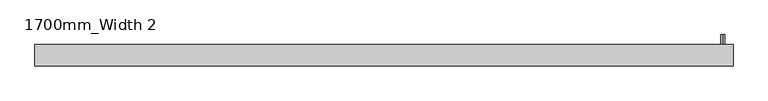
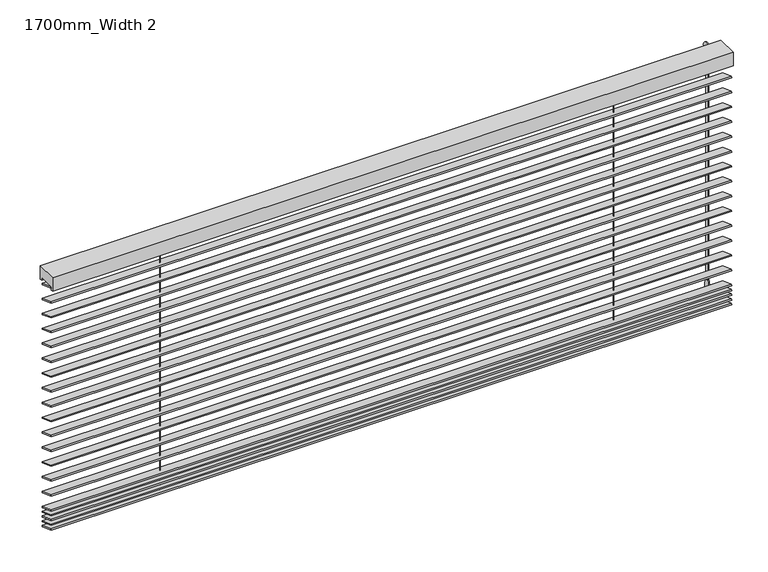
"""IFC4 building model written with IfcOpenShell, lengths in millimetres: proxy geometry, Specialty_Equipment_Venetian_Blind_Half_Down : 1700mm_Width 2."""

from ifc_helpers import new_model, si_unit, point, frame, frame_2d, origin, place, context, project, spatial, polyline, circle_curve, ellipse_curve, trimmed, segment, composite_curve, outline, extrude, source, transform, mapped, element, save
from ifc_brep_helpers import plane_surface, cylinder_surface, revolved_surface, advanced_brep


def proxy_1700mm_width_2_f283f02f(model_context):
    return source(origin(), model_context, "Body", "SolidModel", [
        extrude(outline(polyline([(0.0, 40.0), (1680.0, 40.0), (1680.0, 0.0), (0.0, 0.0), (0.0, 40.0)])), frame((-689.5079376, -65.0532351, 1447.7279746), z_axis=(0.0, 0.3420201433256684, 0.9396926207859085), x_axis=(1.0, 0.0, 0.0)), (0.0, 0.0, 1.0), 3.0625345),
        extrude(outline(polyline([(0.0, 40.0), (1680.0, 40.0), (1680.0, 0.0), (0.0, 0.0), (0.0, 40.0)])), frame((-689.5079376, -65.0532351, 1459.9116214), z_axis=(0.0, 0.3420201433256684, 0.9396926207859085), x_axis=(1.0, 0.0, 0.0)), (0.0, 0.0, 1.0), 3.0625345),
        extrude(outline(polyline([(0.0, 40.0), (1680.0, 40.0), (1680.0, 0.0), (0.0, 0.0), (0.0, 40.0)])), frame((-689.5079376, -65.0532351, 1472.7202682), z_axis=(0.0, 0.3420201433256684, 0.9396926207859085), x_axis=(1.0, 0.0, 0.0)), (0.0, 0.0, 1.0), 3.0625345),
        extrude(outline(polyline([(0.0, 40.0), (1680.0, 40.0), (1680.0, 0.0), (0.0, 0.0), (0.0, 40.0)])), frame((-689.5079376, -65.0532351, 1484.903915), z_axis=(0.0, 0.3420201433256684, 0.9396926207859085), x_axis=(1.0, 0.0, 0.0)), (0.0, 0.0, 1.0), 3.0625345),
        extrude(outline(polyline([(0.0, 40.0), (1680.0, 40.0), (1680.0, 0.0), (0.0, 0.0), (0.0, 40.0)])), frame((-689.5079376, -65.0532351, 2040.2125618), z_axis=(0.0, 0.3420201433256684, 0.9396926207859085), x_axis=(1.0, 0.0, 0.0)), (0.0, 0.0, 1.0), 3.0625345),
        extrude(outline(polyline([(0.0, 40.0), (1680.0, 40.0), (1680.0, 0.0), (0.0, 0.0), (0.0, 40.0)])), frame((-689.5079376, -65.0532351, 2001.4625618), z_axis=(0.0, 0.3420201433256684, 0.9396926207859085), x_axis=(1.0, 0.0, 0.0)), (0.0, 0.0, 1.0), 3.0625345),
        extrude(outline(polyline([(0.0, 40.0), (1680.0, 40.0), (1680.0, 0.0), (0.0, 0.0), (0.0, 40.0)])), frame((-689.5079376, -65.0532351, 1962.7125618), z_axis=(0.0, 0.3420201433256684, 0.9396926207859085), x_axis=(1.0, 0.0, 0.0)), (0.0, 0.0, 1.0), 3.0625345),
        extrude(outline(polyline([(0.0, 40.0), (1680.0, 40.0), (1680.0, 0.0), (0.0, 0.0), (0.0, 40.0)])), frame((-689.5079376, -65.0532351, 1923.9625618), z_axis=(0.0, 0.3420201433256684, 0.9396926207859085), x_axis=(1.0, 0.0, 0.0)), (0.0, 0.0, 1.0), 3.0625345),
        extrude(outline(polyline([(0.0, 40.0), (1680.0, 40.0), (1680.0, 0.0), (0.0, 0.0), (0.0, 40.0)])), frame((-689.5079376, -65.0532351, 1885.2125618), z_axis=(0.0, 0.3420201433256684, 0.9396926207859085), x_axis=(1.0, 0.0, 0.0)), (0.0, 0.0, 1.0), 3.0625345),
        extrude(outline(polyline([(0.0, 40.0), (1680.0, 40.0), (1680.0, 0.0), (0.0, 0.0), (0.0, 40.0)])), frame((-689.5079376, -65.0532351, 1846.4625618), z_axis=(0.0, 0.3420201433256684, 0.9396926207859085), x_axis=(1.0, 0.0, 0.0)), (0.0, 0.0, 1.0), 3.0625345),
        extrude(outline(polyline([(0.0, 40.0), (1680.0, 40.0), (1680.0, 0.0), (0.0, 0.0), (0.0, 40.0)])), frame((-689.5079376, -65.0532351, 1807.7125618), z_axis=(0.0, 0.3420201433256684, 0.9396926207859085), x_axis=(1.0, 0.0, 0.0)), (0.0, 0.0, 1.0), 3.0625345),
        extrude(outline(polyline([(0.0, 40.0), (1680.0, 40.0), (1680.0, 0.0), (0.0, 0.0), (0.0, 40.0)])), frame((-689.5079376, -65.0532351, 1768.9625618), z_axis=(0.0, 0.3420201433256684, 0.9396926207859085), x_axis=(1.0, 0.0, 0.0)), (0.0, 0.0, 1.0), 3.0625345),
        extrude(outline(polyline([(0.0, 40.0), (1680.0, 40.0), (1680.0, 0.0), (0.0, 0.0), (0.0, 40.0)])), frame((-689.5079376, -65.0532351, 1730.2125618), z_axis=(0.0, 0.3420201433256684, 0.9396926207859085), x_axis=(1.0, 0.0, 0.0)), (0.0, 0.0, 1.0), 3.0625345),
        extrude(outline(polyline([(0.0, 40.0), (1680.0, 40.0), (1680.0, 0.0), (0.0, 0.0), (0.0, 40.0)])), frame((-689.5079376, -65.0532351, 1691.4625618), z_axis=(0.0, 0.3420201433256684, 0.9396926207859085), x_axis=(1.0, 0.0, 0.0)), (0.0, 0.0, 1.0), 3.0625345),
        extrude(outline(polyline([(0.0, 40.0), (1680.0, 40.0), (1680.0, 0.0), (0.0, 0.0), (0.0, 40.0)])), frame((-689.5079376, -65.0532351, 1652.7125618), z_axis=(0.0, 0.3420201433256684, 0.9396926207859085), x_axis=(1.0, 0.0, 0.0)), (0.0, 0.0, 1.0), 3.0625345),
        extrude(outline(polyline([(0.0, 40.0), (1680.0, 40.0), (1680.0, 0.0), (0.0, 0.0), (0.0, 40.0)])), frame((-689.5079376, -65.0532351, 1613.9625618), z_axis=(0.0, 0.3420201433256684, 0.9396926207859085), x_axis=(1.0, 0.0, 0.0)), (0.0, 0.0, 1.0), 3.0625345),
        extrude(outline(polyline([(0.0, 40.0), (1680.0, 40.0), (1680.0, 0.0), (0.0, 0.0), (0.0, 40.0)])), frame((-689.5079376, -65.0532351, 1575.2125618), z_axis=(0.0, 0.3420201433256684, 0.9396926207859085), x_axis=(1.0, 0.0, 0.0)), (0.0, 0.0, 1.0), 3.0625345),
        extrude(outline(polyline([(0.0, 40.0), (1680.0, 40.0), (1680.0, 0.0), (0.0, 0.0), (0.0, 40.0)])), frame((-689.5079376, -65.0532351, 1536.4625618), z_axis=(0.0, 0.3420201433256684, 0.9396926207859085), x_axis=(1.0, 0.0, 0.0)), (0.0, 0.0, 1.0), 3.0625345),
        extrude(outline(polyline([(0.0, 40.0), (1680.0, 40.0), (1680.0, 0.0), (0.0, 0.0), (0.0, 40.0)])), frame((-689.5079376, -65.0532351, 1497.7125618), z_axis=(0.0, 0.3420201433256684, 0.9396926207859085), x_axis=(1.0, 0.0, 0.0)), (0.0, 0.0, 1.0), 3.0625345),
        extrude(outline(polyline([(0.0, 40.0), (1680.0, 40.0), (1680.0, 0.0), (0.0, 0.0), (0.0, 40.0)])), frame((-689.5079376, -65.0532351, 2078.9625618), z_axis=(0.0, 0.3420201433256684, 0.9396926207859085), x_axis=(1.0, 0.0, 0.0)), (0.0, 0.0, 1.0), 3.0625345),
        extrude(outline(composite_curve([segment(trimmed(circle_curve(frame_2d((-409.5079376, -45.2119342)), 0.5), [point((-410.0079376, -45.2119342))], [point((-409.0079376, -45.2119342))], False, "CARTESIAN"), True, "CONTINUOUS"), segment(trimmed(circle_curve(frame_2d((-409.5079376, -45.2119342)), 0.5), [point((-409.0079376, -45.2119342))], [point((-410.0079376, -45.2119342))], False, "CARTESIAN"), True, "CONTINUOUS")], self_intersect=False)), frame((0.0, 0.0, 1434.9736305), z_axis=(0.0, 0.0, 1.0), x_axis=(1.0, 0.0, 0.0)), (0.0, 0.0, 1.0), 648.2712578),
        extrude(outline(composite_curve([segment(trimmed(circle_curve(frame_2d((710.4920624, -45.2119342)), 0.5), [point((709.9920624, -45.2119342))], [point((710.9920624, -45.2119342))], False, "CARTESIAN"), True, "CONTINUOUS"), segment(trimmed(circle_curve(frame_2d((710.4920624, -45.2119342)), 0.5), [point((710.9920624, -45.2119342))], [point((709.9920624, -45.2119342))], False, "CARTESIAN"), True, "CONTINUOUS")], self_intersect=False)), frame((0.0, 0.0, 1434.9736305), z_axis=(0.0, 0.0, 1.0), x_axis=(1.0, 0.0, 0.0)), (0.0, 0.0, 1.0), 648.2712578),
        advanced_brep(
        [(965.4920624, -4.7248495, 2091.3243671), (965.4920624, -3.7248495, 2091.3243671), (965.4920624, -2.7248495, 2091.3243671), (965.4920624, -4.7248495, 2076.3243671), (965.4920624, -2.7248495, 2076.3243671), (965.4920624, -6.7248495, 2076.3243671), (965.4920624, -0.7248495, 2076.3243671), (965.4920624, -6.7248495, 1486.909931), (965.4920624, -0.7248495, 1486.909931), (965.4920624, -7.2513368, 1460.0), (965.4920624, -0.1983622, 1460.0), (965.4920624, -3.7248495, 1460.0)],
        [
            (0, 1),
            (1, 2),
            (2, 0, circle_curve(frame((965.4920624, -3.7248495, 2091.3243671), z_axis=(0.0, 0.0, 1.0), x_axis=(0.0, 1.0, 0.0)), 1.0)),
            (0, 2, circle_curve(frame((965.4920624, -3.7248495, 2091.3243671), z_axis=(0.0, 0.0, 1.0), x_axis=(0.0, 1.0, 0.0)), 1.0)),
            (3, 0),
            (2, 4),
            (4, 3, circle_curve(frame((965.4920624, -3.7248495, 2076.3243671), z_axis=(0.0, 0.0, 1.0), x_axis=(0.0, 1.0, 0.0)), 1.0)),
            (3, 4, circle_curve(frame((965.4920624, -3.7248495, 2076.3243671), z_axis=(0.0, 0.0, 1.0), x_axis=(0.0, 1.0, 0.0)), 1.0)),
            (5, 3),
            (4, 6),
            (6, 5, circle_curve(frame((965.4920624, -3.7248495, 2076.3243671), z_axis=(0.0, 0.0, 1.0), x_axis=(0.0, 1.0, 0.0)), 3.0)),
            (5, 6, circle_curve(frame((965.4920624, -3.7248495, 2076.3243671), z_axis=(0.0, 0.0, 1.0), x_axis=(0.0, 1.0, 0.0)), 3.0)),
            (7, 5),
            (6, 8),
            (8, 7, circle_curve(frame((965.4920624, -3.7248495, 1486.909931), z_axis=(0.0, 0.0, 1.0), x_axis=(0.0, 1.0, 0.0)), 3.0)),
            (7, 8, circle_curve(frame((965.4920624, -3.7248495, 1486.909931), z_axis=(0.0, 0.0, 1.0), x_axis=(0.0, 1.0, 0.0)), 3.0)),
            (9, 7, circle_curve(frame((965.4920624, 41.8223072, 1472.5), z_axis=(-1.0, 0.0, 0.0), x_axis=(0.0, 1.0, 0.0)), 50.6406214)),
            (8, 10, circle_curve(frame((965.4920624, -49.2720063, 1472.5), z_axis=(-1.0, 0.0, 0.0), x_axis=(0.0, -1.0, 0.0)), 50.6406214)),
            (10, 9, circle_curve(frame((965.4920624, -3.7248495, 1460.0), z_axis=(0.0, 0.0, 1.0), x_axis=(0.0, 1.0, 0.0)), 3.5264873)),
            (9, 10, circle_curve(frame((965.4920624, -3.7248495, 1460.0), z_axis=(0.0, 0.0, 1.0), x_axis=(0.0, 1.0, 0.0)), 3.5264873)),
            (11, 9),
            (10, 11),
        ],
        [
            plane_surface(frame((965.4920624, -3.7248495, 2091.3243671), z_axis=(0.0, 0.0, 1.0), x_axis=(0.0, 1.0, 0.0))),
            cylinder_surface(frame((965.4920624, -3.7248495, 1191.3243671), z_axis=(0.0, 0.0, -1.0), x_axis=(0.0, 1.0, 0.0)), 1.0),
            plane_surface(frame((965.4920624, -3.7248495, 2076.3243671), z_axis=(0.0, 0.0, 1.0), x_axis=(0.0, 1.0, 0.0))),
            cylinder_surface(frame((965.4920624, -3.7248495, 1191.3243671), z_axis=(0.0, 0.0, -1.0), x_axis=(0.0, 1.0, 0.0)), 3.0),
            revolved_surface(trimmed(ellipse_curve(frame((965.4920624, -49.2720063, 1472.5), z_axis=(-1.0, 0.0, 0.0), x_axis=(0.0, -1.0, 0.0)), 50.6406214, 50.6406214), [point((965.4920624, -0.7248495, 1486.909931))], [point((965.4920624, -0.1983622, 1460.0))], True, "CARTESIAN"), (965.4920624, -3.7248495, 1191.3243671), (0.0, 0.0, -1.0)),
            plane_surface(frame((965.4920624, -3.7248495, 1460.0), z_axis=(0.0, 0.0, -1.0), x_axis=(0.0, 1.0, 0.0))),
        ],
        [
            (0, [[1, 2, 3]]),
            (0, [[-2, -1, 4]]),
            (1, [[5, -3, 6, 7]]),
            (1, [[-6, -4, -5, 8]]),
            (2, [[9, -7, 10, 11]]),
            (2, [[-10, -8, -9, 12]]),
            (3, [[13, -11, 14, 15]]),
            (3, [[-14, -12, -13, 16]]),
            (4, [[17, -15, 18, 19]]),
            (4, [[-18, -16, -17, 20]]),
            (5, [[21, -19, 22]]),
            (5, [[-22, -20, -21]]),
        ],
    ),
        extrude(outline(composite_curve([segment(trimmed(circle_curve(frame_2d((2095.9171213, 965.4920624)), 5.0), [point((2100.9171213, 965.4920624))], [point((2090.9171213, 965.4920624))], False, "CARTESIAN"), True, "CONTINUOUS"), segment(trimmed(circle_curve(frame_2d((2095.9171213, 965.4920624)), 5.0), [point((2090.9171213, 965.4920624))], [point((2100.9171213, 965.4920624))], False, "CARTESIAN"), True, "CONTINUOUS")], self_intersect=False)), frame((0.0, -19.329714, 0.0), z_axis=(0.0, 1.0, 0.0), x_axis=(0.0, 0.0, 1.0)), (0.0, 0.0, 1.0), 23.7809602),
        extrude(outline(polyline([(-19.329714, 2110.0), (-19.329714, 2075.0), (-24.329714, 2075.0), (-24.329714, 2083.2448883), (-66.0941545, 2083.2448883), (-66.0941545, 2075.0), (-71.0941545, 2075.0), (-71.0941545, 2110.0), (-19.329714, 2110.0)])), frame((-689.5079376, 0.0, 0.0), z_axis=(1.0, 0.0, 0.0), x_axis=(0.0, 1.0, 0.0)), (0.0, 0.0, 1.0), 1680.0),
    ])


if __name__ == "__main__":
    model = new_model("IFC4")
    model_context = context("Model", 3, world=origin())
    ifc_project = project(units=[si_unit("LENGTHUNIT", "METRE", prefix="MILLI")], contexts=[model_context])
    site = spatial("IfcSite", under=ifc_project)
    building = spatial("IfcBuilding", under=site)
    placement = place(None, origin())
    proxy_1700mm_width_2_shape = proxy_1700mm_width_2_f283f02f(model_context)
    element("IfcBuildingElementProxy", 1, Name="Specialty_Equipment_Venetian_Blind_Half_Down : 1700mm_Width 2", ObjectType="Specialty_Equipment_Venetian_Blind_Half_Down : 1700mm_Width 2", at=placement, inside=building, context=model_context, shape_type="MappedRepresentation", body=[
        mapped(proxy_1700mm_width_2_shape, transform((0.0, 0.0, 0.0), x_axis=(1.0, 0.0, 0.0), y_axis=(0.0, 1.0, 0.0), z_axis=(0.0, 0.0, 1.0))),
    ])
    save(model, "model.ifc")

# Revit data of these elements
# Type "Specialty_Equipment_Venetian_Blind_Half_Down : 1700mm_Width 2"
#   Keynote = "N10/240"
#   Opening Width = 1700 mm
#   End Offset = 10 mm
#   Blind Length = 1680 mm
#   Blind Fixing Height = 2110 mm
#   Blind Depth = 980 mm
#   Blind Angle = 20.00°
#   Blade Depth = 40 mm
#   No of Blades = 25
#   Material Blind = Wood - Birch
# Element 1 (IfcBuildingElementProxy, "Specialty_Equipment_Venetian_Blind_Half_Down : 1700mm_Width 2")
#   Materials on its faces: "Wood - Birch"
# Materials
#   "Wood - Birch": class "Wood", colour RGB 224 178 126, transparency 0
